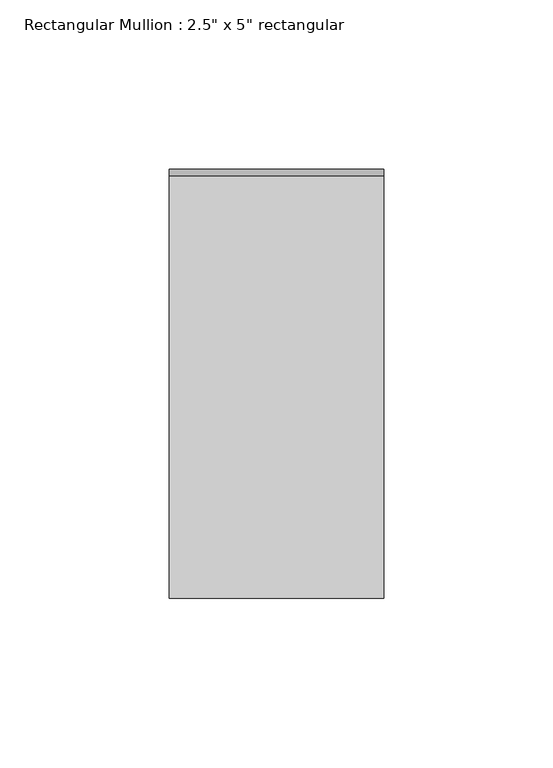
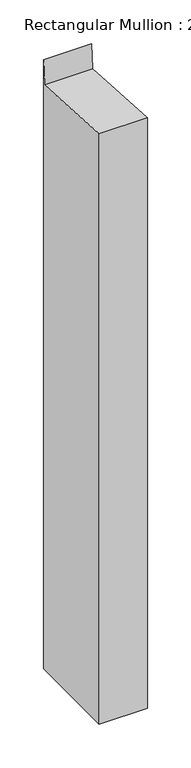
"""IFC4 building model written with IfcOpenShell, lengths in millimetres: member geometry."""

from ifc_helpers import new_model, si_unit, frame, origin, place, context, project, spatial, polyline, outline, extrude, source, transform, mapped, element, save


def member_c839a1ff(model_context):
    return source(origin(), model_context, "Body", "SweptSolid", [
        extrude(outline(polyline([(-63.5, 3.8736342), (61.4149606, -3.8662198), (63.5, 29.7846233), (63.5, -819.15), (-63.5, -819.15), (-63.5, 3.8736342)])), frame((-63.5, 0.0, 0.0), z_axis=(1.0, 0.0, 0.0), x_axis=(0.0, 1.0, 0.0)), (0.0, 0.0, 1.0), 63.5),
    ])


if __name__ == "__main__":
    model = new_model("IFC4")
    model_context = context("Model", 3, world=origin())
    ifc_project = project(units=[si_unit("LENGTHUNIT", "METRE", prefix="MILLI")], contexts=[model_context])
    site = spatial("IfcSite", under=ifc_project)
    building = spatial("IfcBuilding", under=site)
    placement = place(None, origin())
    member_shape = member_c839a1ff(model_context)
    element("IfcMember", 1, ObjectType="Rectangular Mullion : 2.5\" x 5\" rectangular", at=placement, inside=building, context=model_context, shape_type="MappedRepresentation", body=[
        mapped(member_shape, transform((0.0, 0.0, 0.0), x_axis=(1.0, 0.0, 0.0), y_axis=(0.0, 1.0, 0.0), z_axis=(0.0, 0.0, 1.0))),
    ])
    save(model, "model.ifc")

# Revit data of these elements
# Type "Rectangular Mullion : 2.5\" x 5\" rectangular"
#   built-in parameter 1007304 = 0.416667 (stored number, unit not read)
#   built-in parameter 1007301 = 0.104167 (stored number, unit not read)
#   built-in parameter 1007300 = 0.104167 (stored number, unit not read)
# Element 1 (IfcMember, "Rectangular Mullion : 2.5\" x 5\" rectangular")
#   Materials on its faces: "Metal - Aluminum"
# Materials
#   "Metal - Aluminum": class "Metal", colour RGB 247 247 247, transparency 0, Cost = 0
